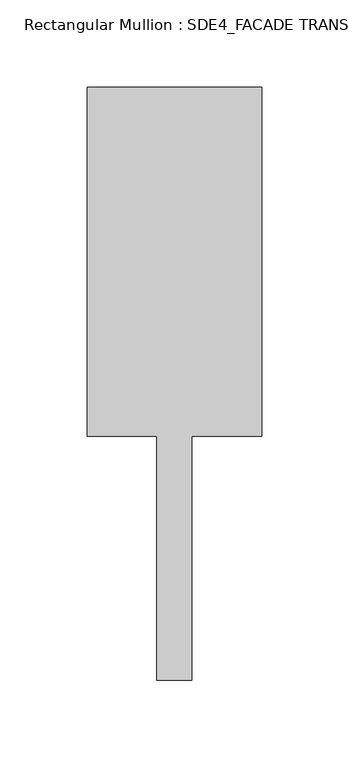
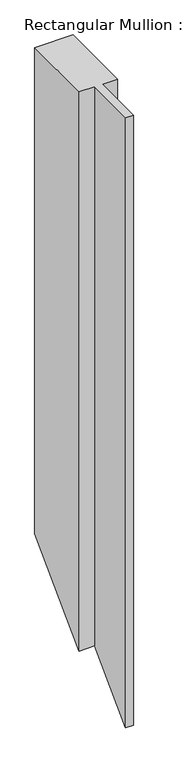
"""IFC4 building model written with IfcOpenShell, lengths in millimetres: member geometry, Rectangular Mullion : SDE4_FACADE TRANSOM TYPE 1."""

from ifc_helpers import new_model, si_unit, origin, place, context, project, spatial, faceted_brep, source, transform, mapped, element, save


def rectangular_mullion_sde4_facade_transom_type_1_be5d2965(model_context):
    return source(origin(), model_context, "Body", "Brep", [
        faceted_brep([(50.0, 132.5, 0.0), (-50.0, 132.5, 0.0), (-50.0, -67.5, 0.0), (-10.0, -67.5, 0.0), (-10.0, -207.5, 0.0), (10.0, -207.5, 0.0), (10.0, -67.5, 0.0), (50.0, -67.5, 0.0), (50.0, 132.5, -1334.0), (-50.0, 132.5, -1334.0), (-50.0, -67.5, -1534.0), (-10.0, -67.5, -1534.0), (-10.0, -207.5, -1674.0), (10.0, -207.5, -1674.0), (10.0, -67.5, -1534.0), (50.0, -67.5, -1534.0)], [[[0, 1, 2, 3, 4, 5, 6, 7]], [[1, 0, 8, 9]], [[2, 1, 9, 10]], [[3, 2, 10, 11]], [[4, 3, 11, 12]], [[5, 4, 12, 13]], [[6, 5, 13, 14]], [[7, 6, 14, 15]], [[0, 7, 15, 8]], [[8, 15, 14, 13, 12, 11, 10, 9]]]),
    ])


if __name__ == "__main__":
    model = new_model("IFC4")
    model_context = context("Model", 3, world=origin())
    ifc_project = project(units=[si_unit("LENGTHUNIT", "METRE", prefix="MILLI")], contexts=[model_context])
    site = spatial("IfcSite", under=ifc_project)
    building = spatial("IfcBuilding", under=site)
    placement = place(None, origin())
    rectangular_mullion_sde4_facade_transom_type_1_shape = rectangular_mullion_sde4_facade_transom_type_1_be5d2965(model_context)
    element("IfcMember", 1, ObjectType="Rectangular Mullion : SDE4_FACADE TRANSOM TYPE 1", at=placement, inside=building, context=model_context, shape_type="MappedRepresentation", body=[
        mapped(rectangular_mullion_sde4_facade_transom_type_1_shape, transform((0.0, 0.0, 0.0), x_axis=(1.0, 0.0, 0.0), y_axis=(0.0, 1.0, 0.0), z_axis=(0.0, 0.0, 1.0))),
    ])
    save(model, "model.ifc")

# Revit data of these elements
# Type "Rectangular Mullion : SDE4_FACADE TRANSOM TYPE 1"
#   built-in parameter 1007322 = 1.11549 (stored number, unit not read)
#   built-in parameter 1007321 = 0.164042 (stored number, unit not read)
#   built-in parameter 1007320 = 0.164042 (stored number, unit not read)
